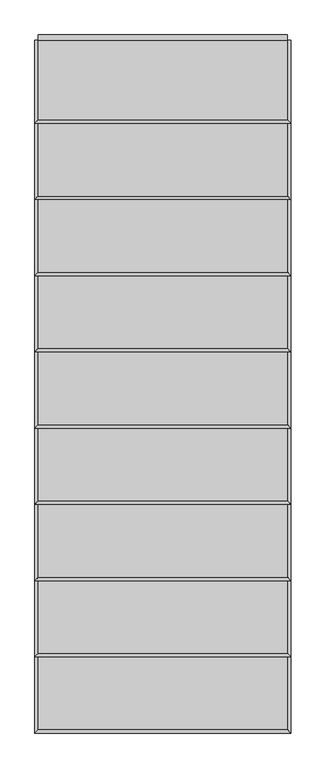
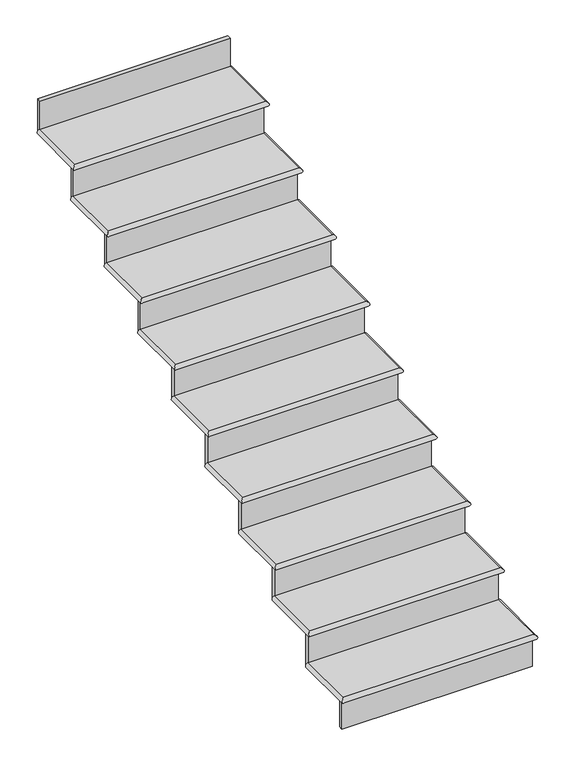
"""IFC4 building model written with IfcOpenShell, lengths in millimetres: stair flight geometry."""

import ifcopenshell
import ifcopenshell.guid

model = None  # the IFC model being written
_history = None  # IfcOwnerHistory: only IFC2X3 demands one
_inside = {}  # id of a spatial element -> (the spatial element, [elements in it])
_under = {}  # id of a project, library or spatial element -> (it, [spatial elements below it])
_declared = {}  # id of a project -> (the project, [libraries it declares])
_typed = {}  # id of a type object -> (the type object, [elements of that type])
_made_of = {}  # id of a material, layer set ... -> (it, [elements and type objects made of it])


def new_model(schema):
    """Start an empty IFC model of exactly this schema.

    Asked for "IFC4X3", IfcOpenShell would pick the latest addendum, in which some entities
    have other attributes; the version numbers below select the first issue.
    IFC2X3 requires an IfcOwnerHistory on every rooted entity: one is made here for all.
    """
    global model, _history
    if schema == "IFC4X3":
        model = ifcopenshell.file(schema_version=(4, 3, 0, 0))
    else:
        model = ifcopenshell.file(schema=schema)
    _inside.clear()
    _under.clear()
    _declared.clear()
    _typed.clear()
    _made_of.clear()
    _history = None
    if model.schema == "IFC2X3":
        org = make("IfcOrganization", Name="unknown")
        user = make(
            "IfcPersonAndOrganization",
            ThePerson=make("IfcPerson", FamilyName="unknown"),
            TheOrganization=org,
        )
        app = make(
            "IfcApplication",
            ApplicationDeveloper=org,
            Version="unknown",
            ApplicationFullName="unknown",
            ApplicationIdentifier="unknown",
        )
        _history = make(
            "IfcOwnerHistory",
            OwningUser=user,
            OwningApplication=app,
            ChangeAction="ADDED",
            CreationDate=0,
        )
    return model


def make(cls, **values):
    """One entity of the class cls with the attributes given. An attribute that is None is left unset."""
    return model.create_entity(
        cls, **{name: value for name, value in values.items() if value is not None}
    )


def rooted(cls, **values):
    """An entity with a GlobalId (a new one), such as an element, a storey or a relation."""
    return make(cls, GlobalId=ifcopenshell.guid.new(), OwnerHistory=_history, **values)


def si_unit(unit_type, name, prefix=None):
    """IfcSIUnit, for example si_unit("LENGTHUNIT", "METRE", prefix="MILLI")."""
    return make("IfcSIUnit", UnitType=unit_type, Prefix=prefix, Name=name)


def assignment(units):
    """IfcUnitAssignment: the units of a project."""
    return None if units is None else make("IfcUnitAssignment", Units=units)


def point(xyz):
    """IfcCartesianPoint."""
    return None if xyz is None else make("IfcCartesianPoint", Coordinates=xyz)


def direction(xyz):
    """IfcDirection."""
    return None if xyz is None else make("IfcDirection", DirectionRatios=xyz)


def frame(location, z_axis=None, x_axis=None):
    """IfcAxis2Placement3D, a coordinate frame: its origin and axes. An axis left out is left unset."""
    return make(
        "IfcAxis2Placement3D",
        Location=point(location),
        Axis=direction(z_axis),
        RefDirection=direction(x_axis),
    )


def origin():
    """The frame at (0, 0, 0) with its axes left unset."""
    return frame((0.0, 0.0, 0.0))


def place(relative_to, where):
    """IfcLocalPlacement: puts the frame where relative to a parent placement (None: the world)."""
    return make(
        "IfcLocalPlacement", PlacementRelTo=relative_to, RelativePlacement=where
    )


def context(
    kind, dimensions, precision=None, world=None, true_north=None, identifier=None
):
    """IfcGeometricRepresentationContext, for example the 3D "Model" context."""
    return make(
        "IfcGeometricRepresentationContext",
        ContextIdentifier=identifier,
        ContextType=kind,
        CoordinateSpaceDimension=dimensions,
        Precision=precision,
        WorldCoordinateSystem=world,
        TrueNorth=true_north,
    )


def project(units=None, contexts=None):
    """IfcProject with its units and contexts."""
    return rooted(
        "IfcProject",
        Name="project",
        RepresentationContexts=contexts,
        UnitsInContext=assignment(units),
    )


def spatial(cls, under=None, at=None, **own):
    """A site, building, storey or space (cls), placed at a placement, below another one or the project."""
    s = rooted(cls, ObjectPlacement=at, **own)
    if under is not None:
        _under.setdefault(under.id(), (under, []))[1].append(s)
    return s


def circle_curve(where, radius):
    """IfcCircle in the frame where."""
    return make("IfcCircle", Position=where, Radius=radius)


def ellipse_curve(where, semi_axis1, semi_axis2):
    """IfcEllipse in the frame where."""
    return make(
        "IfcEllipse", Position=where, SemiAxis1=semi_axis1, SemiAxis2=semi_axis2
    )


def faces_of(points, faces, orient=None, outer=None):
    """IfcFace entities. A face is a list of loops; a loop is a list of indices into points, from 0.

    orient and outer hold one flag for each loop. By default every Orientation is true, the
    first loop of a face is its IfcFaceOuterBound and the others are IfcFaceBound.
    """
    made = []
    for i, loops in enumerate(faces):
        bounds = []
        for j, loop in enumerate(loops):
            is_outer = j == 0 if outer is None else outer[i][j]
            bounds.append(
                make(
                    "IfcFaceOuterBound" if is_outer else "IfcFaceBound",
                    Bound=make("IfcPolyLoop", Polygon=[points[k] for k in loop]),
                    Orientation=True if orient is None else orient[i][j],
                )
            )
        made.append(make("IfcFace", Bounds=bounds))
    return made


def faceted_brep(points, faces, orient=None, outer=None, voids=None):
    """IfcFacetedBrep: a solid bounded by flat faces; with voids (closed shells), ...WithVoids."""
    shared = [point(p) for p in points]
    hull = make("IfcClosedShell", CfsFaces=faces_of(shared, faces, orient, outer))
    if voids is None:
        return make("IfcFacetedBrep", Outer=hull)
    return make(
        "IfcFacetedBrepWithVoids",
        Outer=hull,
        Voids=[
            make(cls, CfsFaces=faces_of(shared, fs, o, b)) for cls, fs, o, b in voids
        ],
    )


def shape(context_of_items, identifier, shape_type, items):
    """IfcShapeRepresentation: the items that make up one representation, for example the "Body"."""
    return make(
        "IfcShapeRepresentation",
        ContextOfItems=context_of_items,
        RepresentationIdentifier=identifier,
        RepresentationType=shape_type,
        Items=items,
    )


def source(mapping_origin, context_of_items, identifier, shape_type, items):
    """IfcRepresentationMap: a shape defined once, which mapped items show again and again."""
    return make(
        "IfcRepresentationMap",
        MappingOrigin=mapping_origin,
        MappedRepresentation=shape(context_of_items, identifier, shape_type, items),
    )


def transform(
    local_origin,
    x_axis=None,
    y_axis=None,
    z_axis=None,
    scale=None,
    scale2=None,
    scale3=None,
    uniform=True,
):
    """IfcCartesianTransformationOperator3D, or its non-uniform kind. x_axis, y_axis, z_axis: its Axis1, 2, 3."""
    if uniform:
        return make(
            "IfcCartesianTransformationOperator3D",
            Axis1=direction(x_axis),
            Axis2=direction(y_axis),
            LocalOrigin=point(local_origin),
            Scale=scale,
            Axis3=direction(z_axis),
        )
    return make(
        "IfcCartesianTransformationOperator3DnonUniform",
        Axis1=direction(x_axis),
        Axis2=direction(y_axis),
        LocalOrigin=point(local_origin),
        Scale=scale,
        Axis3=direction(z_axis),
        Scale2=scale2,
        Scale3=scale3,
    )


def mapped(mapping_source, mapping_target):
    """IfcMappedItem: shows the shape of a source again, moved by a transform."""
    return make(
        "IfcMappedItem", MappingSource=mapping_source, MappingTarget=mapping_target
    )


def made_of(thing, what):
    """Note that an element or type object is made of a material, layer set ...; save() writes the relation."""
    if what is not None:
        _made_of.setdefault(what.id(), (what, []))[1].append(thing)
    return thing


def element(
    cls,
    number,
    at=None,
    inside=None,
    cuts=None,
    type_object=None,
    material=None,
    context=None,
    identifier="Body",
    shape_type=None,
    held_by="IfcProductDefinitionShape",
    body=None,
    shapes=None,
    **own,
):
    """One element of the class cls, such as IfcWall. Its Tag is "e" and its number.

    at: its placement. inside: the storey or other place that contains it. cuts: it is an
    opening in that element (IfcRelVoidsElement). A single representation is given by context,
    identifier, shape_type and body (its items); several are given by shapes. held_by: the class
    of the entity that holds the representations. save() writes the other relations.
    """
    e = rooted(cls, Tag="e%d" % number, ObjectPlacement=at, **own)
    if body is not None:
        shapes = [shape(context, identifier, shape_type, body)]
    if shapes is not None:
        e.Representation = make(held_by, Representations=shapes)
    if inside is not None:
        _inside.setdefault(inside.id(), (inside, []))[1].append(e)
    if cuts is not None:
        rooted(
            "IfcRelVoidsElement", RelatingBuildingElement=cuts, RelatedOpeningElement=e
        )
    if type_object is not None:
        _typed.setdefault(type_object.id(), (type_object, []))[1].append(e)
    return made_of(e, material)


def aggregate(whole, parts):
    """IfcRelAggregates: a whole, such as a stair, and the parts it consists of."""
    return rooted("IfcRelAggregates", RelatingObject=whole, RelatedObjects=parts)


def save(model, path):
    """Write the relations noted so far, then the file.

    IfcRelAggregates (storeys below a building ...), IfcRelContainedInSpatialStructure (elements
    in a storey), IfcRelDefinesByType, IfcRelAssociatesMaterial and IfcRelDeclares: one each for
    every whole, place, type object, material and project.
    """
    for whole, parts in _under.values():
        aggregate(whole, parts)
    for where, things in _inside.values():
        rooted(
            "IfcRelContainedInSpatialStructure",
            RelatedElements=things,
            RelatingStructure=where,
        )
    for kind, things in _typed.values():
        rooted("IfcRelDefinesByType", RelatedObjects=things, RelatingType=kind)
    for what, things in _made_of.values():
        rooted("IfcRelAssociatesMaterial", RelatedObjects=things, RelatingMaterial=what)
    for by, libraries in _declared.values():
        rooted("IfcRelDeclares", RelatingContext=by, RelatedDefinitions=libraries)
    model.write(path)


def plane_surface(at):
    """IfcPlane: the flat surface through the origin of the frame at, square to its z axis."""
    return make("IfcPlane", Position=at)


def cylinder_surface(at, radius):
    """IfcCylindricalSurface: all points at the distance radius from the z axis of the frame at."""
    return make("IfcCylindricalSurface", Position=at, Radius=radius)


def advanced_brep(points, edges, surfaces, faces):
    """IfcAdvancedBrep: a solid bounded by faces that lie on surfaces and meet in shared edges.

    An edge is (start, end): straight between two places in points (the first is 0);
    or (start, end, curve); or (start, end, curve, False) where it runs against its curve.
    A face is (place in surfaces, loops), or (place, loops, False) where it looks against
    its surface's normal. A loop lists edges by number (the first is 1), with a minus sign
    where the edge is run from its end to its start. The first loop is the outer one.
    """
    corners = [point(p) for p in points]
    vertices = [make("IfcVertexPoint", VertexGeometry=c) for c in corners]
    made = []
    for start, end, *more in edges:
        made.append(
            make(
                "IfcEdgeCurve",
                EdgeStart=vertices[start],
                EdgeEnd=vertices[end],
                EdgeGeometry=more[0] if more else make("IfcPolyline", Points=[corners[start], corners[end]]),
                SameSense=more[1] if len(more) > 1 else True,
            )
        )
    hull = []
    for where, loops, *sense in faces:
        bounds = []
        for j, loop in enumerate(loops):
            ring = [make("IfcOrientedEdge", EdgeElement=made[abs(k) - 1], Orientation=k > 0) for k in loop]
            bounds.append(
                make(
                    "IfcFaceOuterBound" if j == 0 else "IfcFaceBound",
                    Bound=make("IfcEdgeLoop", EdgeList=ring),
                    Orientation=True,
                )
            )
        hull.append(make("IfcAdvancedFace", Bounds=bounds, FaceSurface=surfaces[where], SameSense=sense[0] if sense else True))
    return make("IfcAdvancedBrep", Outer=make("IfcClosedShell", CfsFaces=hull))


def stair_flight_efac3296(model_context):
    return source(origin(), model_context, "Body", "SolidModel", [
        advanced_brep(
        [(-6869.5581077, -11168.733999, 143.9333333), (-6869.5581077, -11168.733999, 169.3333333), (-7783.9581077, -11168.733999, 169.3333333), (-7783.9581077, -11168.733999, 143.9333333), (-6869.5581077, -10876.633999, 169.3333333), (-7783.9581077, -10876.633999, 169.3333333), (-7783.9581077, -10876.633999, 143.9333333), (-6869.5581077, -10876.633999, 143.9333333)],
        [
            (0, 1, ellipse_curve(frame((-6869.5581077, -11168.733999, 156.6333333), z_axis=(-0.7071067811865496, -0.7071067811865456, 0.0), x_axis=(0.7071067811865455, -0.7071067811865495, 0.0)), 17.9605122, 12.7)),
            (1, 2),
            (2, 3, ellipse_curve(frame((-7783.9581077, -11168.733999, 156.6333333), z_axis=(0.7071067811865455, -0.7071067811865495, 0.0), x_axis=(0.7071067811865496, 0.7071067811865455, 0.0)), 17.9605122, 12.7)),
            (3, 0),
            (4, 5),
            (5, 2),
            (1, 4),
            (6, 7),
            (7, 0),
            (3, 6),
            (4, 7, circle_curve(frame((-6869.5581077, -10876.633999, 156.6333333), z_axis=(0.0, 1.0, 0.0), x_axis=(-1.0, 0.0, 0.0)), 12.7)),
            (6, 5, circle_curve(frame((-7783.9581077, -10876.633999, 156.6333333), z_axis=(0.0, 1.0, 0.0), x_axis=(1.0, 0.0, 0.0)), 12.7)),
        ],
        [
            cylinder_surface(frame((-6869.5581077, -11168.733999, 156.6333333), z_axis=(1.0, 0.0, 0.0), x_axis=(0.0, 1.0, 0.0)), 12.7),
            plane_surface(frame((-7783.9581077, -10902.033999, 169.3333333), z_axis=(0.0, 0.0, 1.0), x_axis=(0.0, -1.0, 0.0))),
            plane_surface(frame((-7783.9581077, -10902.033999, 143.9333333), z_axis=(0.0, 0.0, -1.0), x_axis=(0.0, 1.0, 0.0))),
            plane_surface(frame((-6869.5581077, -10876.633999, 169.3333333), z_axis=(0.0, 1.0, 0.0), x_axis=(0.0, 0.0, -1.0))),
            cylinder_surface(frame((-6869.5581077, -10876.633999, 156.6333333), z_axis=(0.0, 1.0, 0.0), x_axis=(-1.0, 0.0, 0.0)), 12.7),
            cylinder_surface(frame((-7783.9581077, -11168.733999, 156.6333333), z_axis=(0.0, -1.0, 0.0), x_axis=(1.0, 0.0, 0.0)), 12.7),
        ],
        [
            (0, [[1, 2, 3, 4]]),
            (1, [[5, 6, -2, 7]]),
            (2, [[8, 9, -4, 10]]),
            (3, [[-5, 11, -8, 12]]),
            (4, [[-11, -7, -1, -9]]),
            (5, [[-3, -6, -12, -10]]),
        ],
    ),
        faceted_brep([(-6869.5581077, -11156.033999, 143.9333333), (-6869.5581077, -11156.033999, 0.0), (-6869.5581077, -11136.983999, 0.0), (-6869.5581077, -11136.983999, 143.9333333), (-7783.9581077, -11156.033999, 143.9333333), (-7783.9581077, -11136.983999, 143.9333333), (-7783.9581077, -11136.983999, 0.0), (-7783.9581077, -11156.033999, 0.0)], [[[0, 1, 2, 3]], [[4, 5, 6, 7]], [[1, 0, 4, 7]], [[2, 1, 7, 6]], [[3, 2, 6, 5]], [[0, 3, 5, 4]]]),
        faceted_brep([(-6869.5581077, -10876.633999, 313.2666667), (-6869.5581077, -10876.633999, 143.9333333), (-6869.5581077, -10857.583999, 143.9333333), (-6869.5581077, -10857.583999, 313.2666667), (-7783.9581077, -10876.633999, 313.2666667), (-7783.9581077, -10857.583999, 313.2666667), (-7783.9581077, -10857.583999, 143.9333333), (-7783.9581077, -10876.633999, 143.9333333)], [[[0, 1, 2, 3]], [[4, 5, 6, 7]], [[1, 0, 4, 7]], [[2, 1, 7, 6]], [[3, 2, 6, 5]], [[0, 3, 5, 4]]]),
        advanced_brep(
        [(-6869.5581077, -10597.233999, 338.6666667), (-7783.9581077, -10597.233999, 338.6666667), (-7783.9581077, -10889.333999, 338.6666667), (-6869.5581077, -10889.333999, 338.6666667), (-7783.9581077, -10597.233999, 313.2666667), (-6869.5581077, -10597.233999, 313.2666667), (-6869.5581077, -10889.333999, 313.2666667), (-7783.9581077, -10889.333999, 313.2666667)],
        [
            (0, 1),
            (1, 2),
            (2, 3),
            (3, 0),
            (4, 5),
            (5, 6),
            (6, 7),
            (7, 4),
            (0, 5, circle_curve(frame((-6869.5581077, -10597.233999, 325.9666667), z_axis=(0.0, 1.0, 0.0), x_axis=(-1.0, 0.0, 0.0)), 12.7)),
            (4, 1, circle_curve(frame((-7783.9581077, -10597.233999, 325.9666667), z_axis=(0.0, 1.0, 0.0), x_axis=(1.0, 0.0, 0.0)), 12.7)),
            (6, 3, ellipse_curve(frame((-6869.5581077, -10889.333999, 325.9666667), z_axis=(-0.7071067811865481, -0.7071067811865469, 0.0), x_axis=(0.7071067811865469, -0.7071067811865481, 0.0)), 17.9605122, 12.7)),
            (2, 7, ellipse_curve(frame((-7783.9581077, -10889.333999, 325.9666667), z_axis=(0.7071067811865469, -0.7071067811865481, 0.0), x_axis=(0.7071067811865481, 0.7071067811865468, 0.0)), 17.9605122, 12.7)),
        ],
        [
            plane_surface(frame((-7783.9581077, -10902.033999, 338.6666667), z_axis=(0.0, 0.0, 1.0), x_axis=(0.0, -1.0, 0.0))),
            plane_surface(frame((-7783.9581077, -10902.033999, 313.2666667), z_axis=(0.0, 0.0, -1.0), x_axis=(0.0, 1.0, 0.0))),
            plane_surface(frame((-6869.5581077, -10597.233999, 338.6666667), z_axis=(0.0, 1.0, 0.0), x_axis=(0.0, 0.0, -1.0))),
            cylinder_surface(frame((-6869.5581077, -10889.333999, 325.9666667), z_axis=(1.0, 0.0, 0.0), x_axis=(0.0, 1.0, 0.0)), 12.7),
            cylinder_surface(frame((-6869.5581077, -10597.233999, 325.9666667), z_axis=(0.0, 1.0, 0.0), x_axis=(-1.0, 0.0, 0.0)), 12.7),
            cylinder_surface(frame((-7783.9581077, -10889.333999, 325.9666667), z_axis=(0.0, -1.0, 0.0), x_axis=(1.0, 0.0, 0.0)), 12.7),
        ],
        [
            (0, [[1, 2, 3, 4]]),
            (1, [[5, 6, 7, 8]]),
            (2, [[-1, 9, -5, 10]]),
            (3, [[11, -3, 12, -7]]),
            (4, [[-9, -4, -11, -6]]),
            (5, [[-12, -2, -10, -8]]),
        ],
    ),
        faceted_brep([(-6869.5581077, -10597.233999, 482.6), (-6869.5581077, -10597.233999, 313.2666667), (-6869.5581077, -10578.183999, 313.2666667), (-6869.5581077, -10578.183999, 482.6), (-7783.9581077, -10597.233999, 482.6), (-7783.9581077, -10578.183999, 482.6), (-7783.9581077, -10578.183999, 313.2666667), (-7783.9581077, -10597.233999, 313.2666667)], [[[0, 1, 2, 3]], [[4, 5, 6, 7]], [[1, 0, 4, 7]], [[2, 1, 7, 6]], [[3, 2, 6, 5]], [[0, 3, 5, 4]]]),
        advanced_brep(
        [(-6869.5581077, -10317.833999, 508.0), (-7783.9581077, -10317.833999, 508.0), (-7783.9581077, -10609.933999, 508.0), (-6869.5581077, -10609.933999, 508.0), (-7783.9581077, -10317.833999, 482.6), (-6869.5581077, -10317.833999, 482.6), (-6869.5581077, -10609.933999, 482.6), (-7783.9581077, -10609.933999, 482.6)],
        [
            (0, 1),
            (1, 2),
            (2, 3),
            (3, 0),
            (4, 5),
            (5, 6),
            (6, 7),
            (7, 4),
            (0, 5, circle_curve(frame((-6869.5581077, -10317.833999, 495.3), z_axis=(0.0, 1.0, 0.0), x_axis=(-1.0, 0.0, 0.0)), 12.7)),
            (4, 1, circle_curve(frame((-7783.9581077, -10317.833999, 495.3), z_axis=(0.0, 1.0, 0.0), x_axis=(1.0, 0.0, 0.0)), 12.7)),
            (6, 3, ellipse_curve(frame((-6869.5581077, -10609.933999, 495.3), z_axis=(-0.7071067811865481, -0.7071067811865469, 0.0), x_axis=(0.7071067811865469, -0.7071067811865481, 0.0)), 17.9605122, 12.7)),
            (2, 7, ellipse_curve(frame((-7783.9581077, -10609.933999, 495.3), z_axis=(0.7071067811865469, -0.7071067811865481, 0.0), x_axis=(0.7071067811865481, 0.7071067811865468, 0.0)), 17.9605122, 12.7)),
        ],
        [
            plane_surface(frame((-7783.9581077, -10622.633999, 508.0), z_axis=(0.0, 0.0, 1.0), x_axis=(0.0, -1.0, 0.0))),
            plane_surface(frame((-7783.9581077, -10622.633999, 482.6), z_axis=(0.0, 0.0, -1.0), x_axis=(0.0, 1.0, 0.0))),
            plane_surface(frame((-6869.5581077, -10317.833999, 508.0), z_axis=(0.0, 1.0, 0.0), x_axis=(0.0, 0.0, -1.0))),
            cylinder_surface(frame((-6869.5581077, -10609.933999, 495.3), z_axis=(1.0, 0.0, 0.0), x_axis=(0.0, 1.0, 0.0)), 12.7),
            cylinder_surface(frame((-6869.5581077, -10317.833999, 495.3), z_axis=(0.0, 1.0, 0.0), x_axis=(-1.0, 0.0, 0.0)), 12.7),
            cylinder_surface(frame((-7783.9581077, -10609.933999, 495.3), z_axis=(0.0, -1.0, 0.0), x_axis=(1.0, 0.0, 0.0)), 12.7),
        ],
        [
            (0, [[1, 2, 3, 4]]),
            (1, [[5, 6, 7, 8]]),
            (2, [[-1, 9, -5, 10]]),
            (3, [[11, -3, 12, -7]]),
            (4, [[-9, -4, -11, -6]]),
            (5, [[-12, -2, -10, -8]]),
        ],
    ),
        faceted_brep([(-6869.5581077, -10317.833999, 651.9333333), (-6869.5581077, -10317.833999, 482.6), (-6869.5581077, -10298.783999, 482.6), (-6869.5581077, -10298.783999, 651.9333333), (-7783.9581077, -10317.833999, 651.9333333), (-7783.9581077, -10298.783999, 651.9333333), (-7783.9581077, -10298.783999, 482.6), (-7783.9581077, -10317.833999, 482.6)], [[[0, 1, 2, 3]], [[4, 5, 6, 7]], [[1, 0, 4, 7]], [[2, 1, 7, 6]], [[3, 2, 6, 5]], [[0, 3, 5, 4]]]),
        advanced_brep(
        [(-6869.5581077, -10038.433999, 677.3333333), (-7783.9581077, -10038.433999, 677.3333333), (-7783.9581077, -10330.533999, 677.3333333), (-6869.5581077, -10330.533999, 677.3333333), (-7783.9581077, -10038.433999, 651.9333333), (-6869.5581077, -10038.433999, 651.9333333), (-6869.5581077, -10330.533999, 651.9333333), (-7783.9581077, -10330.533999, 651.9333333)],
        [
            (0, 1),
            (1, 2),
            (2, 3),
            (3, 0),
            (4, 5),
            (5, 6),
            (6, 7),
            (7, 4),
            (0, 5, circle_curve(frame((-6869.5581077, -10038.433999, 664.6333333), z_axis=(0.0, 1.0, 0.0), x_axis=(-1.0, 0.0, 0.0)), 12.7)),
            (4, 1, circle_curve(frame((-7783.9581077, -10038.433999, 664.6333333), z_axis=(0.0, 1.0, 0.0), x_axis=(1.0, 0.0, 0.0)), 12.7)),
            (6, 3, ellipse_curve(frame((-6869.5581077, -10330.533999, 664.6333333), z_axis=(-0.7071067811865481, -0.7071067811865469, 0.0), x_axis=(0.7071067811865469, -0.7071067811865481, 0.0)), 17.9605122, 12.7)),
            (2, 7, ellipse_curve(frame((-7783.9581077, -10330.533999, 664.6333333), z_axis=(0.7071067811865469, -0.7071067811865481, 0.0), x_axis=(0.7071067811865481, 0.7071067811865468, 0.0)), 17.9605122, 12.7)),
        ],
        [
            plane_surface(frame((-7783.9581077, -10343.233999, 677.3333333), z_axis=(0.0, 0.0, 1.0), x_axis=(0.0, -1.0, 0.0))),
            plane_surface(frame((-7783.9581077, -10343.233999, 651.9333333), z_axis=(0.0, 0.0, -1.0), x_axis=(0.0, 1.0, 0.0))),
            plane_surface(frame((-6869.5581077, -10038.433999, 677.3333333), z_axis=(0.0, 1.0, 0.0), x_axis=(0.0, 0.0, -1.0))),
            cylinder_surface(frame((-6869.5581077, -10330.533999, 664.6333333), z_axis=(1.0, 0.0, 0.0), x_axis=(0.0, 1.0, 0.0)), 12.7),
            cylinder_surface(frame((-6869.5581077, -10038.433999, 664.6333333), z_axis=(0.0, 1.0, 0.0), x_axis=(-1.0, 0.0, 0.0)), 12.7),
            cylinder_surface(frame((-7783.9581077, -10330.533999, 664.6333333), z_axis=(0.0, -1.0, 0.0), x_axis=(1.0, 0.0, 0.0)), 12.7),
        ],
        [
            (0, [[1, 2, 3, 4]]),
            (1, [[5, 6, 7, 8]]),
            (2, [[-1, 9, -5, 10]]),
            (3, [[11, -3, 12, -7]]),
            (4, [[-9, -4, -11, -6]]),
            (5, [[-12, -2, -10, -8]]),
        ],
    ),
        faceted_brep([(-6869.5581077, -10038.433999, 821.2666667), (-6869.5581077, -10038.433999, 651.9333333), (-6869.5581077, -10019.383999, 651.9333333), (-6869.5581077, -10019.383999, 821.2666667), (-7783.9581077, -10038.433999, 821.2666667), (-7783.9581077, -10019.383999, 821.2666667), (-7783.9581077, -10019.383999, 651.9333333), (-7783.9581077, -10038.433999, 651.9333333)], [[[0, 1, 2, 3]], [[4, 5, 6, 7]], [[1, 0, 4, 7]], [[2, 1, 7, 6]], [[3, 2, 6, 5]], [[0, 3, 5, 4]]]),
        advanced_brep(
        [(-6869.5581077, -9759.033999, 846.6666667), (-7783.9581077, -9759.033999, 846.6666667), (-7783.9581077, -10051.133999, 846.6666667), (-6869.5581077, -10051.133999, 846.6666667), (-7783.9581077, -9759.033999, 821.2666667), (-6869.5581077, -9759.033999, 821.2666667), (-6869.5581077, -10051.133999, 821.2666667), (-7783.9581077, -10051.133999, 821.2666667)],
        [
            (0, 1),
            (1, 2),
            (2, 3),
            (3, 0),
            (4, 5),
            (5, 6),
            (6, 7),
            (7, 4),
            (0, 5, circle_curve(frame((-6869.5581077, -9759.033999, 833.9666667), z_axis=(0.0, 1.0, 0.0), x_axis=(-1.0, 0.0, 0.0)), 12.7)),
            (4, 1, circle_curve(frame((-7783.9581077, -9759.033999, 833.9666667), z_axis=(0.0, 1.0, 0.0), x_axis=(1.0, 0.0, 0.0)), 12.7)),
            (6, 3, ellipse_curve(frame((-6869.5581077, -10051.133999, 833.9666667), z_axis=(-0.7071067811865481, -0.7071067811865469, 0.0), x_axis=(0.7071067811865469, -0.7071067811865481, 0.0)), 17.9605122, 12.7)),
            (2, 7, ellipse_curve(frame((-7783.9581077, -10051.133999, 833.9666667), z_axis=(0.7071067811865469, -0.7071067811865481, 0.0), x_axis=(0.7071067811865481, 0.7071067811865468, 0.0)), 17.9605122, 12.7)),
        ],
        [
            plane_surface(frame((-7783.9581077, -10063.833999, 846.6666667), z_axis=(0.0, 0.0, 1.0), x_axis=(0.0, -1.0, 0.0))),
            plane_surface(frame((-7783.9581077, -10063.833999, 821.2666667), z_axis=(0.0, 0.0, -1.0), x_axis=(0.0, 1.0, 0.0))),
            plane_surface(frame((-6869.5581077, -9759.033999, 846.6666667), z_axis=(0.0, 1.0, 0.0), x_axis=(0.0, 0.0, -1.0))),
            cylinder_surface(frame((-6869.5581077, -10051.133999, 833.9666667), z_axis=(1.0, 0.0, 0.0), x_axis=(0.0, 1.0, 0.0)), 12.7),
            cylinder_surface(frame((-6869.5581077, -9759.033999, 833.9666667), z_axis=(0.0, 1.0, 0.0), x_axis=(-1.0, 0.0, 0.0)), 12.7),
            cylinder_surface(frame((-7783.9581077, -10051.133999, 833.9666667), z_axis=(0.0, -1.0, 0.0), x_axis=(1.0, 0.0, 0.0)), 12.7),
        ],
        [
            (0, [[1, 2, 3, 4]]),
            (1, [[5, 6, 7, 8]]),
            (2, [[-1, 9, -5, 10]]),
            (3, [[11, -3, 12, -7]]),
            (4, [[-9, -4, -11, -6]]),
            (5, [[-12, -2, -10, -8]]),
        ],
    ),
        faceted_brep([(-6869.5581077, -9759.033999, 990.6), (-6869.5581077, -9759.033999, 821.2666667), (-6869.5581077, -9739.983999, 821.2666667), (-6869.5581077, -9739.983999, 990.6), (-7783.9581077, -9759.033999, 990.6), (-7783.9581077, -9739.983999, 990.6), (-7783.9581077, -9739.983999, 821.2666667), (-7783.9581077, -9759.033999, 821.2666667)], [[[0, 1, 2, 3]], [[4, 5, 6, 7]], [[1, 0, 4, 7]], [[2, 1, 7, 6]], [[3, 2, 6, 5]], [[0, 3, 5, 4]]]),
        advanced_brep(
        [(-6869.5581077, -9479.633999, 1016.0), (-7783.9581077, -9479.633999, 1016.0), (-7783.9581077, -9771.733999, 1016.0), (-6869.5581077, -9771.733999, 1016.0), (-7783.9581077, -9479.633999, 990.6), (-6869.5581077, -9479.633999, 990.6), (-6869.5581077, -9771.733999, 990.6), (-7783.9581077, -9771.733999, 990.6)],
        [
            (0, 1),
            (1, 2),
            (2, 3),
            (3, 0),
            (4, 5),
            (5, 6),
            (6, 7),
            (7, 4),
            (0, 5, circle_curve(frame((-6869.5581077, -9479.633999, 1003.3), z_axis=(0.0, 1.0, 0.0), x_axis=(-1.0, 0.0, 0.0)), 12.7)),
            (4, 1, circle_curve(frame((-7783.9581077, -9479.633999, 1003.3), z_axis=(0.0, 1.0, 0.0), x_axis=(1.0, 0.0, 0.0)), 12.7)),
            (6, 3, ellipse_curve(frame((-6869.5581077, -9771.733999, 1003.3), z_axis=(-0.7071067811865481, -0.7071067811865469, 0.0), x_axis=(0.7071067811865469, -0.7071067811865481, 0.0)), 17.9605122, 12.7)),
            (2, 7, ellipse_curve(frame((-7783.9581077, -9771.733999, 1003.3), z_axis=(0.7071067811865469, -0.7071067811865481, 0.0), x_axis=(0.7071067811865481, 0.7071067811865468, 0.0)), 17.9605122, 12.7)),
        ],
        [
            plane_surface(frame((-7783.9581077, -9784.433999, 1016.0), z_axis=(0.0, 0.0, 1.0), x_axis=(0.0, -1.0, 0.0))),
            plane_surface(frame((-7783.9581077, -9784.433999, 990.6), z_axis=(0.0, 0.0, -1.0), x_axis=(0.0, 1.0, 0.0))),
            plane_surface(frame((-6869.5581077, -9479.633999, 1016.0), z_axis=(0.0, 1.0, 0.0), x_axis=(0.0, 0.0, -1.0))),
            cylinder_surface(frame((-6869.5581077, -9771.733999, 1003.3), z_axis=(1.0, 0.0, 0.0), x_axis=(0.0, 1.0, 0.0)), 12.7),
            cylinder_surface(frame((-6869.5581077, -9479.633999, 1003.3), z_axis=(0.0, 1.0, 0.0), x_axis=(-1.0, 0.0, 0.0)), 12.7),
            cylinder_surface(frame((-7783.9581077, -9771.733999, 1003.3), z_axis=(0.0, -1.0, 0.0), x_axis=(1.0, 0.0, 0.0)), 12.7),
        ],
        [
            (0, [[1, 2, 3, 4]]),
            (1, [[5, 6, 7, 8]]),
            (2, [[-1, 9, -5, 10]]),
            (3, [[11, -3, 12, -7]]),
            (4, [[-9, -4, -11, -6]]),
            (5, [[-12, -2, -10, -8]]),
        ],
    ),
        faceted_brep([(-6869.5581077, -9479.633999, 1159.9333333), (-6869.5581077, -9479.633999, 990.6), (-6869.5581077, -9460.583999, 990.6), (-6869.5581077, -9460.583999, 1159.9333333), (-7783.9581077, -9479.633999, 1159.9333333), (-7783.9581077, -9460.583999, 1159.9333333), (-7783.9581077, -9460.583999, 990.6), (-7783.9581077, -9479.633999, 990.6)], [[[0, 1, 2, 3]], [[4, 5, 6, 7]], [[1, 0, 4, 7]], [[2, 1, 7, 6]], [[3, 2, 6, 5]], [[0, 3, 5, 4]]]),
        advanced_brep(
        [(-6869.5581077, -9200.233999, 1185.3333333), (-7783.9581077, -9200.233999, 1185.3333333), (-7783.9581077, -9492.333999, 1185.3333333), (-6869.5581077, -9492.333999, 1185.3333333), (-7783.9581077, -9200.233999, 1159.9333333), (-6869.5581077, -9200.233999, 1159.9333333), (-6869.5581077, -9492.333999, 1159.9333333), (-7783.9581077, -9492.333999, 1159.9333333)],
        [
            (0, 1),
            (1, 2),
            (2, 3),
            (3, 0),
            (4, 5),
            (5, 6),
            (6, 7),
            (7, 4),
            (0, 5, circle_curve(frame((-6869.5581077, -9200.233999, 1172.6333333), z_axis=(0.0, 1.0, 0.0), x_axis=(-1.0, 0.0, 0.0)), 12.7)),
            (4, 1, circle_curve(frame((-7783.9581077, -9200.233999, 1172.6333333), z_axis=(0.0, 1.0, 0.0), x_axis=(1.0, 0.0, 0.0)), 12.7)),
            (6, 3, ellipse_curve(frame((-6869.5581077, -9492.333999, 1172.6333333), z_axis=(-0.7071067811865481, -0.7071067811865469, 0.0), x_axis=(0.7071067811865469, -0.7071067811865481, 0.0)), 17.9605122, 12.7)),
            (2, 7, ellipse_curve(frame((-7783.9581077, -9492.333999, 1172.6333333), z_axis=(0.7071067811865469, -0.7071067811865481, 0.0), x_axis=(0.7071067811865481, 0.7071067811865468, 0.0)), 17.9605122, 12.7)),
        ],
        [
            plane_surface(frame((-7783.9581077, -9505.033999, 1185.3333333), z_axis=(0.0, 0.0, 1.0), x_axis=(0.0, -1.0, 0.0))),
            plane_surface(frame((-7783.9581077, -9505.033999, 1159.9333333), z_axis=(0.0, 0.0, -1.0), x_axis=(0.0, 1.0, 0.0))),
            plane_surface(frame((-6869.5581077, -9200.233999, 1185.3333333), z_axis=(0.0, 1.0, 0.0), x_axis=(0.0, 0.0, -1.0))),
            cylinder_surface(frame((-6869.5581077, -9492.333999, 1172.6333333), z_axis=(1.0, 0.0, 0.0), x_axis=(0.0, 1.0, 0.0)), 12.7),
            cylinder_surface(frame((-6869.5581077, -9200.233999, 1172.6333333), z_axis=(0.0, 1.0, 0.0), x_axis=(-1.0, 0.0, 0.0)), 12.7),
            cylinder_surface(frame((-7783.9581077, -9492.333999, 1172.6333333), z_axis=(0.0, -1.0, 0.0), x_axis=(1.0, 0.0, 0.0)), 12.7),
        ],
        [
            (0, [[1, 2, 3, 4]]),
            (1, [[5, 6, 7, 8]]),
            (2, [[-1, 9, -5, 10]]),
            (3, [[11, -3, 12, -7]]),
            (4, [[-9, -4, -11, -6]]),
            (5, [[-12, -2, -10, -8]]),
        ],
    ),
        faceted_brep([(-6869.5581077, -9200.233999, 1329.2666667), (-6869.5581077, -9200.233999, 1159.9333333), (-6869.5581077, -9181.183999, 1159.9333333), (-6869.5581077, -9181.183999, 1329.2666667), (-7783.9581077, -9200.233999, 1329.2666667), (-7783.9581077, -9181.183999, 1329.2666667), (-7783.9581077, -9181.183999, 1159.9333333), (-7783.9581077, -9200.233999, 1159.9333333)], [[[0, 1, 2, 3]], [[4, 5, 6, 7]], [[1, 0, 4, 7]], [[2, 1, 7, 6]], [[3, 2, 6, 5]], [[0, 3, 5, 4]]]),
        advanced_brep(
        [(-6869.5581077, -8920.833999, 1354.6666667), (-7783.9581077, -8920.833999, 1354.6666667), (-7783.9581077, -9212.933999, 1354.6666667), (-6869.5581077, -9212.933999, 1354.6666667), (-7783.9581077, -8920.833999, 1329.2666667), (-6869.5581077, -8920.833999, 1329.2666667), (-6869.5581077, -9212.933999, 1329.2666667), (-7783.9581077, -9212.933999, 1329.2666667)],
        [
            (0, 1),
            (1, 2),
            (2, 3),
            (3, 0),
            (4, 5),
            (5, 6),
            (6, 7),
            (7, 4),
            (0, 5, circle_curve(frame((-6869.5581077, -8920.833999, 1341.9666667), z_axis=(0.0, 1.0, 0.0), x_axis=(-1.0, 0.0, 0.0)), 12.7)),
            (4, 1, circle_curve(frame((-7783.9581077, -8920.833999, 1341.9666667), z_axis=(0.0, 1.0, 0.0), x_axis=(1.0, 0.0, 0.0)), 12.7)),
            (6, 3, ellipse_curve(frame((-6869.5581077, -9212.933999, 1341.9666667), z_axis=(-0.7071067811865481, -0.7071067811865469, 0.0), x_axis=(0.7071067811865469, -0.7071067811865481, 0.0)), 17.9605122, 12.7)),
            (2, 7, ellipse_curve(frame((-7783.9581077, -9212.933999, 1341.9666667), z_axis=(0.7071067811865469, -0.7071067811865481, 0.0), x_axis=(0.7071067811865481, 0.7071067811865468, 0.0)), 17.9605122, 12.7)),
        ],
        [
            plane_surface(frame((-7783.9581077, -9225.633999, 1354.6666667), z_axis=(0.0, 0.0, 1.0), x_axis=(0.0, -1.0, 0.0))),
            plane_surface(frame((-7783.9581077, -9225.633999, 1329.2666667), z_axis=(0.0, 0.0, -1.0), x_axis=(0.0, 1.0, 0.0))),
            plane_surface(frame((-6869.5581077, -8920.833999, 1354.6666667), z_axis=(0.0, 1.0, 0.0), x_axis=(0.0, 0.0, -1.0))),
            cylinder_surface(frame((-6869.5581077, -9212.933999, 1341.9666667), z_axis=(1.0, 0.0, 0.0), x_axis=(0.0, 1.0, 0.0)), 12.7),
            cylinder_surface(frame((-6869.5581077, -8920.833999, 1341.9666667), z_axis=(0.0, 1.0, 0.0), x_axis=(-1.0, 0.0, 0.0)), 12.7),
            cylinder_surface(frame((-7783.9581077, -9212.933999, 1341.9666667), z_axis=(0.0, -1.0, 0.0), x_axis=(1.0, 0.0, 0.0)), 12.7),
        ],
        [
            (0, [[1, 2, 3, 4]]),
            (1, [[5, 6, 7, 8]]),
            (2, [[-1, 9, -5, 10]]),
            (3, [[11, -3, 12, -7]]),
            (4, [[-9, -4, -11, -6]]),
            (5, [[-12, -2, -10, -8]]),
        ],
    ),
        faceted_brep([(-6869.5581077, -8641.433999, 1667.9333333), (-6869.5581077, -8641.433999, 1498.6), (-6869.5581077, -8622.383999, 1498.6), (-6869.5581077, -8622.383999, 1667.9333333), (-7783.9581077, -8641.433999, 1667.9333333), (-7783.9581077, -8622.383999, 1667.9333333), (-7783.9581077, -8622.383999, 1498.6), (-7783.9581077, -8641.433999, 1498.6)], [[[0, 1, 2, 3]], [[4, 5, 6, 7]], [[1, 0, 4, 7]], [[2, 1, 7, 6]], [[3, 2, 6, 5]], [[0, 3, 5, 4]]]),
        faceted_brep([(-6869.5581077, -8920.833999, 1498.6), (-6869.5581077, -8920.833999, 1329.2666667), (-6869.5581077, -8901.783999, 1329.2666667), (-6869.5581077, -8901.783999, 1498.6), (-7783.9581077, -8920.833999, 1498.6), (-7783.9581077, -8901.783999, 1498.6), (-7783.9581077, -8901.783999, 1329.2666667), (-7783.9581077, -8920.833999, 1329.2666667)], [[[0, 1, 2, 3]], [[4, 5, 6, 7]], [[1, 0, 4, 7]], [[2, 1, 7, 6]], [[3, 2, 6, 5]], [[0, 3, 5, 4]]]),
        advanced_brep(
        [(-6869.5581077, -8641.433999, 1524.0), (-7783.9581077, -8641.433999, 1524.0), (-7783.9581077, -8666.833999, 1524.0), (-7783.9581077, -8933.533999, 1524.0), (-6869.5581077, -8933.533999, 1524.0), (-6869.5581077, -8666.833999, 1524.0), (-7783.9581077, -8641.433999, 1498.6), (-6869.5581077, -8641.433999, 1498.6), (-6869.5581077, -8666.833999, 1498.6), (-6869.5581077, -8933.533999, 1498.6), (-7783.9581077, -8933.533999, 1498.6), (-7783.9581077, -8666.833999, 1498.6)],
        [
            (0, 1),
            (1, 2),
            (2, 3),
            (3, 4),
            (4, 5),
            (5, 0),
            (6, 7),
            (7, 8),
            (8, 9),
            (9, 10),
            (10, 11),
            (11, 6),
            (0, 7, circle_curve(frame((-6869.5581077, -8641.433999, 1511.3), z_axis=(0.0, 1.0, 0.0), x_axis=(-1.0, 0.0, 0.0)), 12.7)),
            (6, 1, circle_curve(frame((-7783.9581077, -8641.433999, 1511.3), z_axis=(0.0, 1.0, 0.0), x_axis=(1.0, 0.0, 0.0)), 12.7)),
            (9, 4, ellipse_curve(frame((-6869.5581077, -8933.533999, 1511.3), z_axis=(-0.7071067811865475, -0.7071067811865475, 0.0), x_axis=(0.7071067811865476, -0.7071067811865474, 0.0)), 17.9605122, 12.7)),
            (3, 10, ellipse_curve(frame((-7783.9581077, -8933.533999, 1511.3), z_axis=(0.7071067811865469, -0.7071067811865481, 0.0), x_axis=(0.7071067811865481, 0.7071067811865469, 0.0)), 17.9605122, 12.7)),
        ],
        [
            plane_surface(frame((-7783.9581077, -8666.833999, 1524.0), z_axis=(0.0, 0.0, 1.0), x_axis=(0.0, -1.0, 0.0))),
            plane_surface(frame((-7783.9581077, -8666.833999, 1498.6), z_axis=(0.0, 0.0, -1.0), x_axis=(0.0, 1.0, 0.0))),
            plane_surface(frame((-6869.5581077, -8641.433999, 1524.0), z_axis=(0.0, 1.0, 0.0), x_axis=(0.0, 0.0, -1.0))),
            cylinder_surface(frame((-6869.5581077, -8933.533999, 1511.3), z_axis=(1.0, 0.0, 0.0), x_axis=(0.0, 1.0, 0.0)), 12.7),
            cylinder_surface(frame((-6869.5581077, -8641.433999, 1511.3), z_axis=(0.0, 1.0, 0.0), x_axis=(-1.0, 0.0, 0.0)), 12.7),
            cylinder_surface(frame((-7783.9581077, -8933.533999, 1511.3), z_axis=(0.0, -1.0, 0.0), x_axis=(1.0, 0.0, 0.0)), 12.7),
        ],
        [
            (0, [[1, 2, 3, 4, 5, 6]]),
            (1, [[7, 8, 9, 10, 11, 12]]),
            (2, [[-1, 13, -7, 14]]),
            (3, [[15, -4, 16, -10]]),
            (4, [[-13, -6, -5, -15, -9, -8]]),
            (5, [[-16, -3, -2, -14, -12, -11]]),
        ],
    ),
    ])


if __name__ == "__main__":
    model = new_model("IFC4")
    model_context = context("Model", 3, world=origin())
    ifc_project = project(units=[si_unit("LENGTHUNIT", "METRE", prefix="MILLI")], contexts=[model_context])
    site = spatial("IfcSite", under=ifc_project)
    building = spatial("IfcBuilding", under=site)
    placement = place(None, origin())
    stair_flight_shape = stair_flight_efac3296(model_context)
    element("IfcStairFlight", 1, at=placement, inside=building, context=model_context, shape_type="MappedRepresentation", body=[
        mapped(stair_flight_shape, transform((0.0, 0.0, 0.0), x_axis=(1.0, 0.0, 0.0), y_axis=(0.0, 1.0, 0.0), z_axis=(0.0, 0.0, 1.0))),
    ])
    save(model, "model.ifc")

# Revit data of these elements
# Element 1 (IfcStairFlight)
#   Materials on its faces: "Wood - Cherry"
# Materials
#   "Wood - Cherry": class "Unassigned", colour RGB 226 177 128, transparency 0
